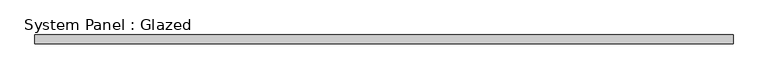
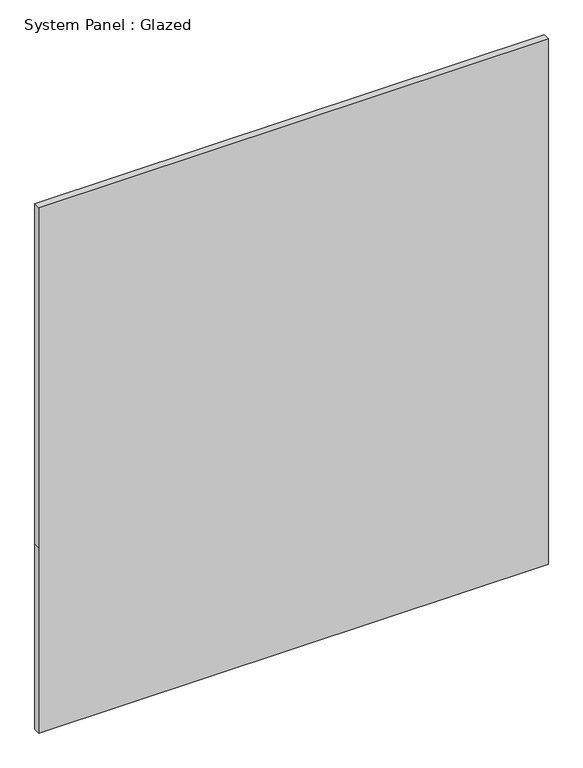
"""IFC4 building model written with IfcOpenShell, lengths in millimetres: plate geometry, System Panel : Glazed."""

from ifc_helpers import new_model, si_unit, frame, origin, place, context, project, spatial, polyline, outline, extrude, source, transform, mapped, element, save


def system_panel_glazed_1e38db9b(model_context):
    return source(origin(), model_context, "Body", "SweptSolid", [
        extrude(outline(polyline([(0.0, -975.0000002), (0.0, 975.0000002), (750.0, 975.0000002), (2125.0, 975.0000002), (2125.0, -975.0000002), (750.0, -975.0000002), (0.0, -975.0000002)])), frame((0.0, 24.5, 0.0), z_axis=(0.0, 1.0, 0.0), x_axis=(0.0, 0.0, 1.0)), (0.0, 0.0, 1.0), 25.0),
    ])


if __name__ == "__main__":
    model = new_model("IFC4")
    model_context = context("Model", 3, world=origin())
    ifc_project = project(units=[si_unit("LENGTHUNIT", "METRE", prefix="MILLI")], contexts=[model_context])
    site = spatial("IfcSite", under=ifc_project)
    building = spatial("IfcBuilding", under=site)
    placement = place(None, origin())
    system_panel_glazed_shape = system_panel_glazed_1e38db9b(model_context)
    element("IfcPlate", 1, ObjectType="System Panel : Glazed", at=placement, inside=building, context=model_context, shape_type="MappedRepresentation", body=[
        mapped(system_panel_glazed_shape, transform((0.0, 0.0, 0.0), x_axis=(1.0, 0.0, 0.0), y_axis=(0.0, 1.0, 0.0), z_axis=(0.0, 0.0, 1.0))),
    ])
    save(model, "model.ifc")

# Revit data of these elements
# Element 1 (IfcPlate, "System Panel : Glazed")
#   Materials on its faces: "Glass"
# Materials
#   "Glass": class "Glass", colour RGB 0 128 192, transparency 0.9
